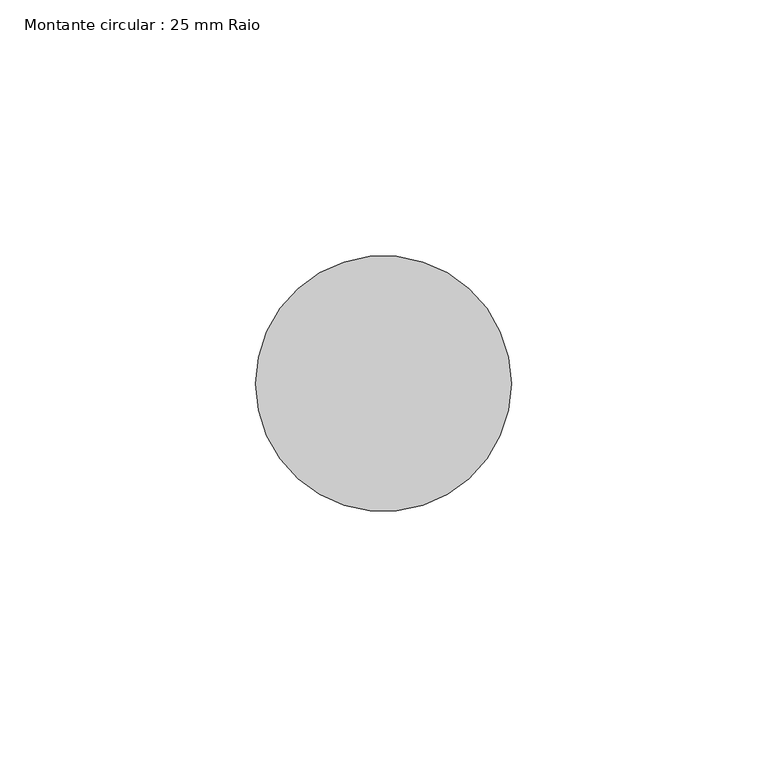
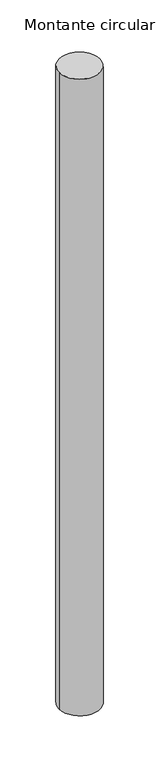
"""IFC4 building model written with IfcOpenShell, lengths in millimetres: member geometry, Montante circular : 25 mm Raio."""

import ifcopenshell
import ifcopenshell.guid

model = None  # the IFC model being written
_history = None  # IfcOwnerHistory: only IFC2X3 demands one
_inside = {}  # id of a spatial element -> (the spatial element, [elements in it])
_under = {}  # id of a project, library or spatial element -> (it, [spatial elements below it])
_declared = {}  # id of a project -> (the project, [libraries it declares])
_typed = {}  # id of a type object -> (the type object, [elements of that type])
_made_of = {}  # id of a material, layer set ... -> (it, [elements and type objects made of it])


def new_model(schema):
    """Start an empty IFC model of exactly this schema.

    Asked for "IFC4X3", IfcOpenShell would pick the latest addendum, in which some entities
    have other attributes; the version numbers below select the first issue.
    IFC2X3 requires an IfcOwnerHistory on every rooted entity: one is made here for all.
    """
    global model, _history
    if schema == "IFC4X3":
        model = ifcopenshell.file(schema_version=(4, 3, 0, 0))
    else:
        model = ifcopenshell.file(schema=schema)
    _inside.clear()
    _under.clear()
    _declared.clear()
    _typed.clear()
    _made_of.clear()
    _history = None
    if model.schema == "IFC2X3":
        org = make("IfcOrganization", Name="unknown")
        user = make(
            "IfcPersonAndOrganization",
            ThePerson=make("IfcPerson", FamilyName="unknown"),
            TheOrganization=org,
        )
        app = make(
            "IfcApplication",
            ApplicationDeveloper=org,
            Version="unknown",
            ApplicationFullName="unknown",
            ApplicationIdentifier="unknown",
        )
        _history = make(
            "IfcOwnerHistory",
            OwningUser=user,
            OwningApplication=app,
            ChangeAction="ADDED",
            CreationDate=0,
        )
    return model


def make(cls, **values):
    """One entity of the class cls with the attributes given. An attribute that is None is left unset."""
    return model.create_entity(
        cls, **{name: value for name, value in values.items() if value is not None}
    )


def rooted(cls, **values):
    """An entity with a GlobalId (a new one), such as an element, a storey or a relation."""
    return make(cls, GlobalId=ifcopenshell.guid.new(), OwnerHistory=_history, **values)


def si_unit(unit_type, name, prefix=None):
    """IfcSIUnit, for example si_unit("LENGTHUNIT", "METRE", prefix="MILLI")."""
    return make("IfcSIUnit", UnitType=unit_type, Prefix=prefix, Name=name)


def assignment(units):
    """IfcUnitAssignment: the units of a project."""
    return None if units is None else make("IfcUnitAssignment", Units=units)


def point(xyz):
    """IfcCartesianPoint."""
    return None if xyz is None else make("IfcCartesianPoint", Coordinates=xyz)


def direction(xyz):
    """IfcDirection."""
    return None if xyz is None else make("IfcDirection", DirectionRatios=xyz)


def frame(location, z_axis=None, x_axis=None):
    """IfcAxis2Placement3D, a coordinate frame: its origin and axes. An axis left out is left unset."""
    return make(
        "IfcAxis2Placement3D",
        Location=point(location),
        Axis=direction(z_axis),
        RefDirection=direction(x_axis),
    )


def frame_2d(location, x_axis=None):
    """IfcAxis2Placement2D, a coordinate frame in the plane: its origin and x axis."""
    return make(
        "IfcAxis2Placement2D", Location=point(location), RefDirection=direction(x_axis)
    )


def origin():
    """The frame at (0, 0, 0) with its axes left unset."""
    return frame((0.0, 0.0, 0.0))


def origin_2d():
    """The frame at (0, 0) in the plane with its x axis left unset."""
    return frame_2d((0.0, 0.0))


def place(relative_to, where):
    """IfcLocalPlacement: puts the frame where relative to a parent placement (None: the world)."""
    return make(
        "IfcLocalPlacement", PlacementRelTo=relative_to, RelativePlacement=where
    )


def context(
    kind, dimensions, precision=None, world=None, true_north=None, identifier=None
):
    """IfcGeometricRepresentationContext, for example the 3D "Model" context."""
    return make(
        "IfcGeometricRepresentationContext",
        ContextIdentifier=identifier,
        ContextType=kind,
        CoordinateSpaceDimension=dimensions,
        Precision=precision,
        WorldCoordinateSystem=world,
        TrueNorth=true_north,
    )


def project(units=None, contexts=None):
    """IfcProject with its units and contexts."""
    return rooted(
        "IfcProject",
        Name="project",
        RepresentationContexts=contexts,
        UnitsInContext=assignment(units),
    )


def spatial(cls, under=None, at=None, **own):
    """A site, building, storey or space (cls), placed at a placement, below another one or the project."""
    s = rooted(cls, ObjectPlacement=at, **own)
    if under is not None:
        _under.setdefault(under.id(), (under, []))[1].append(s)
    return s


def circle_curve(where, radius):
    """IfcCircle in the frame where."""
    return make("IfcCircle", Position=where, Radius=radius)


def trimmed(basis, trim1, trim2, sense, master):
    """IfcTrimmedCurve: the piece of a basis curve between two trims."""
    return make(
        "IfcTrimmedCurve",
        BasisCurve=basis,
        Trim1=trim1,
        Trim2=trim2,
        SenseAgreement=sense,
        MasterRepresentation=master,
    )


def segment(curve, same_sense, transition):
    """IfcCompositeCurveSegment."""
    return make(
        "IfcCompositeCurveSegment",
        Transition=transition,
        SameSense=same_sense,
        ParentCurve=curve,
    )


def composite_curve(segments, self_intersect=None):
    """IfcCompositeCurve: segments joined end to end."""
    return make("IfcCompositeCurve", Segments=segments, SelfIntersect=self_intersect)


def outline(outer, holes=None, kind="AREA"):
    """IfcArbitraryClosedProfileDef: a profile drawn as a closed curve; with holes, ...WithVoids."""
    if holes is None:
        return make("IfcArbitraryClosedProfileDef", ProfileType=kind, OuterCurve=outer)
    return make(
        "IfcArbitraryProfileDefWithVoids",
        ProfileType=kind,
        OuterCurve=outer,
        InnerCurves=holes,
    )


def extrude(swept, where, along, depth):
    """IfcExtrudedAreaSolid: the profile swept, set in the frame where, extruded along a direction by depth."""
    return make(
        "IfcExtrudedAreaSolid",
        SweptArea=swept,
        Position=where,
        ExtrudedDirection=direction(along),
        Depth=depth,
    )


def shape(context_of_items, identifier, shape_type, items):
    """IfcShapeRepresentation: the items that make up one representation, for example the "Body"."""
    return make(
        "IfcShapeRepresentation",
        ContextOfItems=context_of_items,
        RepresentationIdentifier=identifier,
        RepresentationType=shape_type,
        Items=items,
    )


def source(mapping_origin, context_of_items, identifier, shape_type, items):
    """IfcRepresentationMap: a shape defined once, which mapped items show again and again."""
    return make(
        "IfcRepresentationMap",
        MappingOrigin=mapping_origin,
        MappedRepresentation=shape(context_of_items, identifier, shape_type, items),
    )


def transform(
    local_origin,
    x_axis=None,
    y_axis=None,
    z_axis=None,
    scale=None,
    scale2=None,
    scale3=None,
    uniform=True,
):
    """IfcCartesianTransformationOperator3D, or its non-uniform kind. x_axis, y_axis, z_axis: its Axis1, 2, 3."""
    if uniform:
        return make(
            "IfcCartesianTransformationOperator3D",
            Axis1=direction(x_axis),
            Axis2=direction(y_axis),
            LocalOrigin=point(local_origin),
            Scale=scale,
            Axis3=direction(z_axis),
        )
    return make(
        "IfcCartesianTransformationOperator3DnonUniform",
        Axis1=direction(x_axis),
        Axis2=direction(y_axis),
        LocalOrigin=point(local_origin),
        Scale=scale,
        Axis3=direction(z_axis),
        Scale2=scale2,
        Scale3=scale3,
    )


def mapped(mapping_source, mapping_target):
    """IfcMappedItem: shows the shape of a source again, moved by a transform."""
    return make(
        "IfcMappedItem", MappingSource=mapping_source, MappingTarget=mapping_target
    )


def made_of(thing, what):
    """Note that an element or type object is made of a material, layer set ...; save() writes the relation."""
    if what is not None:
        _made_of.setdefault(what.id(), (what, []))[1].append(thing)
    return thing


def element(
    cls,
    number,
    at=None,
    inside=None,
    cuts=None,
    type_object=None,
    material=None,
    context=None,
    identifier="Body",
    shape_type=None,
    held_by="IfcProductDefinitionShape",
    body=None,
    shapes=None,
    **own,
):
    """One element of the class cls, such as IfcWall. Its Tag is "e" and its number.

    at: its placement. inside: the storey or other place that contains it. cuts: it is an
    opening in that element (IfcRelVoidsElement). A single representation is given by context,
    identifier, shape_type and body (its items); several are given by shapes. held_by: the class
    of the entity that holds the representations. save() writes the other relations.
    """
    e = rooted(cls, Tag="e%d" % number, ObjectPlacement=at, **own)
    if body is not None:
        shapes = [shape(context, identifier, shape_type, body)]
    if shapes is not None:
        e.Representation = make(held_by, Representations=shapes)
    if inside is not None:
        _inside.setdefault(inside.id(), (inside, []))[1].append(e)
    if cuts is not None:
        rooted(
            "IfcRelVoidsElement", RelatingBuildingElement=cuts, RelatedOpeningElement=e
        )
    if type_object is not None:
        _typed.setdefault(type_object.id(), (type_object, []))[1].append(e)
    return made_of(e, material)


def aggregate(whole, parts):
    """IfcRelAggregates: a whole, such as a stair, and the parts it consists of."""
    return rooted("IfcRelAggregates", RelatingObject=whole, RelatedObjects=parts)


def save(model, path):
    """Write the relations noted so far, then the file.

    IfcRelAggregates (storeys below a building ...), IfcRelContainedInSpatialStructure (elements
    in a storey), IfcRelDefinesByType, IfcRelAssociatesMaterial and IfcRelDeclares: one each for
    every whole, place, type object, material and project.
    """
    for whole, parts in _under.values():
        aggregate(whole, parts)
    for where, things in _inside.values():
        rooted(
            "IfcRelContainedInSpatialStructure",
            RelatedElements=things,
            RelatingStructure=where,
        )
    for kind, things in _typed.values():
        rooted("IfcRelDefinesByType", RelatedObjects=things, RelatingType=kind)
    for what, things in _made_of.values():
        rooted("IfcRelAssociatesMaterial", RelatedObjects=things, RelatingMaterial=what)
    for by, libraries in _declared.values():
        rooted("IfcRelDeclares", RelatingContext=by, RelatedDefinitions=libraries)
    model.write(path)


def montante_circular_25_mm_raio_603051cb(model_context):
    return source(origin(), model_context, "Body", "SweptSolid", [
        extrude(outline(composite_curve([segment(trimmed(circle_curve(origin_2d(), 25.0), [point((25.0, 0.0))], [point((-25.0, 0.0))], False, "CARTESIAN"), True, "CONTINUOUS"), segment(trimmed(circle_curve(origin_2d(), 25.0), [point((-25.0, 0.0))], [point((25.0, 0.0))], False, "CARTESIAN"), True, "CONTINUOUS")], self_intersect=False)), frame((0.0, 0.0, -822.7451606), z_axis=(0.0, 0.0, 1.0), x_axis=(1.0, 0.0, 0.0)), (0.0, 0.0, 1.0), 822.7451606),
    ])


if __name__ == "__main__":
    model = new_model("IFC4")
    model_context = context("Model", 3, world=origin())
    ifc_project = project(units=[si_unit("LENGTHUNIT", "METRE", prefix="MILLI")], contexts=[model_context])
    site = spatial("IfcSite", under=ifc_project)
    building = spatial("IfcBuilding", under=site)
    placement = place(None, origin())
    montante_circular_25_mm_raio_shape = montante_circular_25_mm_raio_603051cb(model_context)
    element("IfcMember", 1, ObjectType="Montante circular : 25 mm Raio", at=placement, inside=building, context=model_context, shape_type="MappedRepresentation", body=[
        mapped(montante_circular_25_mm_raio_shape, transform((0.0, 0.0, 0.0), x_axis=(1.0, 0.0, 0.0), y_axis=(0.0, 1.0, 0.0), z_axis=(0.0, 0.0, 1.0))),
    ])
    save(model, "model.ifc")

# Revit data of these elements
# Type "Montante circular : 25 mm Raio"
#   built-in parameter 1007350 = 0.082021 (stored number, unit not read)
# Element 1 (IfcMember, "Montante circular : 25 mm Raio")
#   Materials on its faces: "Alumín."
# Materials
#   "Alumín.": class "Metal", colour RGB 247 247 247, transparency 0, Description = "Alumín. 6061", Cost = 0
